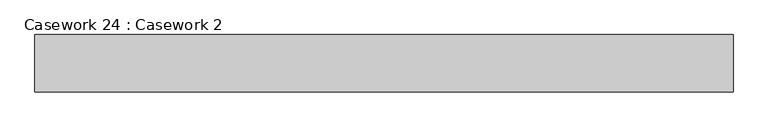
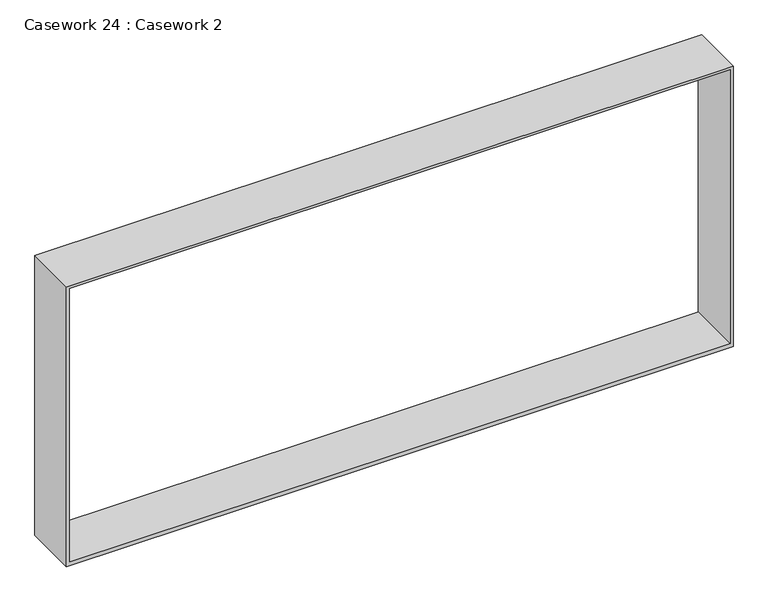
"""IFC4 building model written with IfcOpenShell, lengths in millimetres: furniture geometry, Casework 24 : Casework 2."""

from ifc_helpers import new_model, si_unit, frame, origin, place, context, project, spatial, polyline, outline, extrude, source, transform, mapped, element, save


def casework_24_casework_2_4cfab9a8(model_context):
    return source(origin(), model_context, "Body", "SweptSolid", [
        extrude(outline(polyline([(3048.0, -58223.6551606), (609.6, -58223.6551606), (609.6, -52737.2551606), (3048.0, -52737.2551606), (3048.0, -58223.6551606)]), holes=[polyline([(3024.850107, -58198.2551606), (3024.850107, -52762.6551606), (643.13302, -52762.6551606), (643.13302, -58198.2551606), (3024.850107, -58198.2551606)])]), frame((0.0, 285614.3720148, 0.0), z_axis=(0.0, 1.0, 0.0), x_axis=(0.0, 0.0, 1.0)), (0.0, 0.0, 1.0), 450.1962661),
    ])


if __name__ == "__main__":
    model = new_model("IFC4")
    model_context = context("Model", 3, world=origin())
    ifc_project = project(units=[si_unit("LENGTHUNIT", "METRE", prefix="MILLI")], contexts=[model_context])
    site = spatial("IfcSite", under=ifc_project)
    building = spatial("IfcBuilding", under=site)
    placement = place(None, origin())
    casework_24_casework_2_shape = casework_24_casework_2_4cfab9a8(model_context)
    element("IfcFurniture", 1, ObjectType="Casework 24 : Casework 2", at=placement, inside=building, context=model_context, shape_type="MappedRepresentation", body=[
        mapped(casework_24_casework_2_shape, transform((0.0, 0.0, 0.0), x_axis=(1.0, 0.0, 0.0), y_axis=(0.0, 1.0, 0.0), z_axis=(0.0, 0.0, 1.0))),
    ])
    save(model, "model.ifc")

# Revit data of these elements
# Element 1 (IfcFurniture, "Casework 24 : Casework 2")
#   Materials on its faces: "Dark metal"
# Materials
#   "Dark metal": class "Generic", colour RGB 44 29 29, transparency 0, Cost = 0
